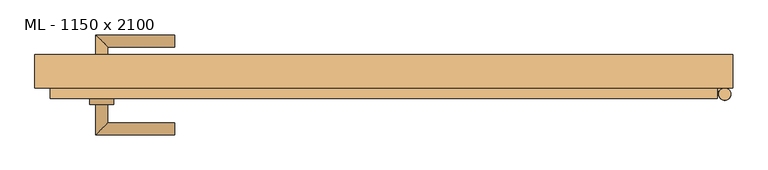
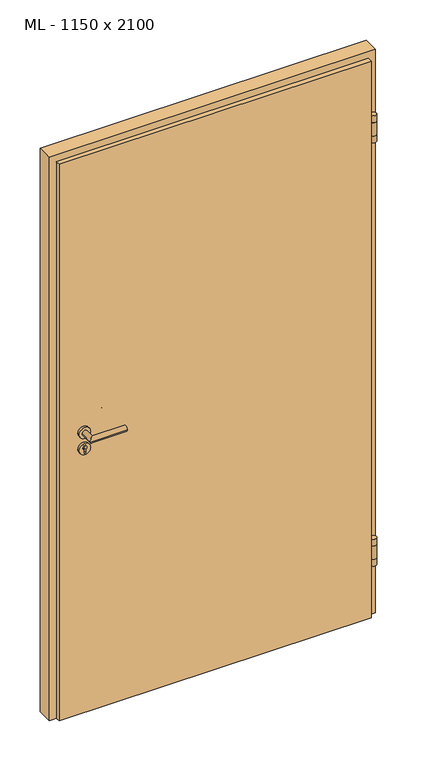
"""IFC4 building model written with IfcOpenShell, lengths in millimetres: door geometry, TU DF 1 - Pfostenstock Falztüre : ML - 1150 x 2100."""

import ifcopenshell
import ifcopenshell.guid

model = None  # the IFC model being written
_history = None  # IfcOwnerHistory: only IFC2X3 demands one
_inside = {}  # id of a spatial element -> (the spatial element, [elements in it])
_under = {}  # id of a project, library or spatial element -> (it, [spatial elements below it])
_declared = {}  # id of a project -> (the project, [libraries it declares])
_typed = {}  # id of a type object -> (the type object, [elements of that type])
_made_of = {}  # id of a material, layer set ... -> (it, [elements and type objects made of it])


def new_model(schema):
    """Start an empty IFC model of exactly this schema.

    Asked for "IFC4X3", IfcOpenShell would pick the latest addendum, in which some entities
    have other attributes; the version numbers below select the first issue.
    IFC2X3 requires an IfcOwnerHistory on every rooted entity: one is made here for all.
    """
    global model, _history
    if schema == "IFC4X3":
        model = ifcopenshell.file(schema_version=(4, 3, 0, 0))
    else:
        model = ifcopenshell.file(schema=schema)
    _inside.clear()
    _under.clear()
    _declared.clear()
    _typed.clear()
    _made_of.clear()
    _history = None
    if model.schema == "IFC2X3":
        org = make("IfcOrganization", Name="unknown")
        user = make(
            "IfcPersonAndOrganization",
            ThePerson=make("IfcPerson", FamilyName="unknown"),
            TheOrganization=org,
        )
        app = make(
            "IfcApplication",
            ApplicationDeveloper=org,
            Version="unknown",
            ApplicationFullName="unknown",
            ApplicationIdentifier="unknown",
        )
        _history = make(
            "IfcOwnerHistory",
            OwningUser=user,
            OwningApplication=app,
            ChangeAction="ADDED",
            CreationDate=0,
        )
    return model


def make(cls, **values):
    """One entity of the class cls with the attributes given. An attribute that is None is left unset."""
    return model.create_entity(
        cls, **{name: value for name, value in values.items() if value is not None}
    )


def rooted(cls, **values):
    """An entity with a GlobalId (a new one), such as an element, a storey or a relation."""
    return make(cls, GlobalId=ifcopenshell.guid.new(), OwnerHistory=_history, **values)


def si_unit(unit_type, name, prefix=None):
    """IfcSIUnit, for example si_unit("LENGTHUNIT", "METRE", prefix="MILLI")."""
    return make("IfcSIUnit", UnitType=unit_type, Prefix=prefix, Name=name)


def assignment(units):
    """IfcUnitAssignment: the units of a project."""
    return None if units is None else make("IfcUnitAssignment", Units=units)


def point(xyz):
    """IfcCartesianPoint."""
    return None if xyz is None else make("IfcCartesianPoint", Coordinates=xyz)


def direction(xyz):
    """IfcDirection."""
    return None if xyz is None else make("IfcDirection", DirectionRatios=xyz)


def frame(location, z_axis=None, x_axis=None):
    """IfcAxis2Placement3D, a coordinate frame: its origin and axes. An axis left out is left unset."""
    return make(
        "IfcAxis2Placement3D",
        Location=point(location),
        Axis=direction(z_axis),
        RefDirection=direction(x_axis),
    )


def frame_2d(location, x_axis=None):
    """IfcAxis2Placement2D, a coordinate frame in the plane: its origin and x axis."""
    return make(
        "IfcAxis2Placement2D", Location=point(location), RefDirection=direction(x_axis)
    )


def origin():
    """The frame at (0, 0, 0) with its axes left unset."""
    return frame((0.0, 0.0, 0.0))


def place(relative_to, where):
    """IfcLocalPlacement: puts the frame where relative to a parent placement (None: the world)."""
    return make(
        "IfcLocalPlacement", PlacementRelTo=relative_to, RelativePlacement=where
    )


def context(
    kind, dimensions, precision=None, world=None, true_north=None, identifier=None
):
    """IfcGeometricRepresentationContext, for example the 3D "Model" context."""
    return make(
        "IfcGeometricRepresentationContext",
        ContextIdentifier=identifier,
        ContextType=kind,
        CoordinateSpaceDimension=dimensions,
        Precision=precision,
        WorldCoordinateSystem=world,
        TrueNorth=true_north,
    )


def project(units=None, contexts=None):
    """IfcProject with its units and contexts."""
    return rooted(
        "IfcProject",
        Name="project",
        RepresentationContexts=contexts,
        UnitsInContext=assignment(units),
    )


def spatial(cls, under=None, at=None, **own):
    """A site, building, storey or space (cls), placed at a placement, below another one or the project."""
    s = rooted(cls, ObjectPlacement=at, **own)
    if under is not None:
        _under.setdefault(under.id(), (under, []))[1].append(s)
    return s


def polyline(points):
    """IfcPolyline through the points."""
    return make("IfcPolyline", Points=[point(p) for p in points])


def circle_curve(where, radius):
    """IfcCircle in the frame where."""
    return make("IfcCircle", Position=where, Radius=radius)


def ellipse_curve(where, semi_axis1, semi_axis2):
    """IfcEllipse in the frame where."""
    return make(
        "IfcEllipse", Position=where, SemiAxis1=semi_axis1, SemiAxis2=semi_axis2
    )


def trimmed(basis, trim1, trim2, sense, master):
    """IfcTrimmedCurve: the piece of a basis curve between two trims."""
    return make(
        "IfcTrimmedCurve",
        BasisCurve=basis,
        Trim1=trim1,
        Trim2=trim2,
        SenseAgreement=sense,
        MasterRepresentation=master,
    )


def segment(curve, same_sense, transition):
    """IfcCompositeCurveSegment."""
    return make(
        "IfcCompositeCurveSegment",
        Transition=transition,
        SameSense=same_sense,
        ParentCurve=curve,
    )


def composite_curve(segments, self_intersect=None):
    """IfcCompositeCurve: segments joined end to end."""
    return make("IfcCompositeCurve", Segments=segments, SelfIntersect=self_intersect)


def outline(outer, holes=None, kind="AREA"):
    """IfcArbitraryClosedProfileDef: a profile drawn as a closed curve; with holes, ...WithVoids."""
    if holes is None:
        return make("IfcArbitraryClosedProfileDef", ProfileType=kind, OuterCurve=outer)
    return make(
        "IfcArbitraryProfileDefWithVoids",
        ProfileType=kind,
        OuterCurve=outer,
        InnerCurves=holes,
    )


def extrude(swept, where, along, depth):
    """IfcExtrudedAreaSolid: the profile swept, set in the frame where, extruded along a direction by depth."""
    return make(
        "IfcExtrudedAreaSolid",
        SweptArea=swept,
        Position=where,
        ExtrudedDirection=direction(along),
        Depth=depth,
    )


def faces_of(points, faces, orient=None, outer=None):
    """IfcFace entities. A face is a list of loops; a loop is a list of indices into points, from 0.

    orient and outer hold one flag for each loop. By default every Orientation is true, the
    first loop of a face is its IfcFaceOuterBound and the others are IfcFaceBound.
    """
    made = []
    for i, loops in enumerate(faces):
        bounds = []
        for j, loop in enumerate(loops):
            is_outer = j == 0 if outer is None else outer[i][j]
            bounds.append(
                make(
                    "IfcFaceOuterBound" if is_outer else "IfcFaceBound",
                    Bound=make("IfcPolyLoop", Polygon=[points[k] for k in loop]),
                    Orientation=True if orient is None else orient[i][j],
                )
            )
        made.append(make("IfcFace", Bounds=bounds))
    return made


def faceted_brep(points, faces, orient=None, outer=None, voids=None):
    """IfcFacetedBrep: a solid bounded by flat faces; with voids (closed shells), ...WithVoids."""
    shared = [point(p) for p in points]
    hull = make("IfcClosedShell", CfsFaces=faces_of(shared, faces, orient, outer))
    if voids is None:
        return make("IfcFacetedBrep", Outer=hull)
    return make(
        "IfcFacetedBrepWithVoids",
        Outer=hull,
        Voids=[
            make(cls, CfsFaces=faces_of(shared, fs, o, b)) for cls, fs, o, b in voids
        ],
    )


def shape(context_of_items, identifier, shape_type, items):
    """IfcShapeRepresentation: the items that make up one representation, for example the "Body"."""
    return make(
        "IfcShapeRepresentation",
        ContextOfItems=context_of_items,
        RepresentationIdentifier=identifier,
        RepresentationType=shape_type,
        Items=items,
    )


def source(mapping_origin, context_of_items, identifier, shape_type, items):
    """IfcRepresentationMap: a shape defined once, which mapped items show again and again."""
    return make(
        "IfcRepresentationMap",
        MappingOrigin=mapping_origin,
        MappedRepresentation=shape(context_of_items, identifier, shape_type, items),
    )


def transform(
    local_origin,
    x_axis=None,
    y_axis=None,
    z_axis=None,
    scale=None,
    scale2=None,
    scale3=None,
    uniform=True,
):
    """IfcCartesianTransformationOperator3D, or its non-uniform kind. x_axis, y_axis, z_axis: its Axis1, 2, 3."""
    if uniform:
        return make(
            "IfcCartesianTransformationOperator3D",
            Axis1=direction(x_axis),
            Axis2=direction(y_axis),
            LocalOrigin=point(local_origin),
            Scale=scale,
            Axis3=direction(z_axis),
        )
    return make(
        "IfcCartesianTransformationOperator3DnonUniform",
        Axis1=direction(x_axis),
        Axis2=direction(y_axis),
        LocalOrigin=point(local_origin),
        Scale=scale,
        Axis3=direction(z_axis),
        Scale2=scale2,
        Scale3=scale3,
    )


def mapped(mapping_source, mapping_target):
    """IfcMappedItem: shows the shape of a source again, moved by a transform."""
    return make(
        "IfcMappedItem", MappingSource=mapping_source, MappingTarget=mapping_target
    )


def made_of(thing, what):
    """Note that an element or type object is made of a material, layer set ...; save() writes the relation."""
    if what is not None:
        _made_of.setdefault(what.id(), (what, []))[1].append(thing)
    return thing


def element(
    cls,
    number,
    at=None,
    inside=None,
    cuts=None,
    type_object=None,
    material=None,
    context=None,
    identifier="Body",
    shape_type=None,
    held_by="IfcProductDefinitionShape",
    body=None,
    shapes=None,
    **own,
):
    """One element of the class cls, such as IfcWall. Its Tag is "e" and its number.

    at: its placement. inside: the storey or other place that contains it. cuts: it is an
    opening in that element (IfcRelVoidsElement). A single representation is given by context,
    identifier, shape_type and body (its items); several are given by shapes. held_by: the class
    of the entity that holds the representations. save() writes the other relations.
    """
    e = rooted(cls, Tag="e%d" % number, ObjectPlacement=at, **own)
    if body is not None:
        shapes = [shape(context, identifier, shape_type, body)]
    if shapes is not None:
        e.Representation = make(held_by, Representations=shapes)
    if inside is not None:
        _inside.setdefault(inside.id(), (inside, []))[1].append(e)
    if cuts is not None:
        rooted(
            "IfcRelVoidsElement", RelatingBuildingElement=cuts, RelatedOpeningElement=e
        )
    if type_object is not None:
        _typed.setdefault(type_object.id(), (type_object, []))[1].append(e)
    return made_of(e, material)


def aggregate(whole, parts):
    """IfcRelAggregates: a whole, such as a stair, and the parts it consists of."""
    return rooted("IfcRelAggregates", RelatingObject=whole, RelatedObjects=parts)


def save(model, path):
    """Write the relations noted so far, then the file.

    IfcRelAggregates (storeys below a building ...), IfcRelContainedInSpatialStructure (elements
    in a storey), IfcRelDefinesByType, IfcRelAssociatesMaterial and IfcRelDeclares: one each for
    every whole, place, type object, material and project.
    """
    for whole, parts in _under.values():
        aggregate(whole, parts)
    for where, things in _inside.values():
        rooted(
            "IfcRelContainedInSpatialStructure",
            RelatedElements=things,
            RelatingStructure=where,
        )
    for kind, things in _typed.values():
        rooted("IfcRelDefinesByType", RelatedObjects=things, RelatingType=kind)
    for what, things in _made_of.values():
        rooted("IfcRelAssociatesMaterial", RelatedObjects=things, RelatingMaterial=what)
    for by, libraries in _declared.values():
        rooted("IfcRelDeclares", RelatingContext=by, RelatedDefinitions=libraries)
    model.write(path)


def plane_surface(at):
    """IfcPlane: the flat surface through the origin of the frame at, square to its z axis."""
    return make("IfcPlane", Position=at)


def cylinder_surface(at, radius):
    """IfcCylindricalSurface: all points at the distance radius from the z axis of the frame at."""
    return make("IfcCylindricalSurface", Position=at, Radius=radius)


def advanced_brep(points, edges, surfaces, faces):
    """IfcAdvancedBrep: a solid bounded by faces that lie on surfaces and meet in shared edges.

    An edge is (start, end): straight between two places in points (the first is 0);
    or (start, end, curve); or (start, end, curve, False) where it runs against its curve.
    A face is (place in surfaces, loops), or (place, loops, False) where it looks against
    its surface's normal. A loop lists edges by number (the first is 1), with a minus sign
    where the edge is run from its end to its start. The first loop is the outer one.
    """
    corners = [point(p) for p in points]
    vertices = [make("IfcVertexPoint", VertexGeometry=c) for c in corners]
    made = []
    for start, end, *more in edges:
        made.append(
            make(
                "IfcEdgeCurve",
                EdgeStart=vertices[start],
                EdgeEnd=vertices[end],
                EdgeGeometry=more[0] if more else make("IfcPolyline", Points=[corners[start], corners[end]]),
                SameSense=more[1] if len(more) > 1 else True,
            )
        )
    hull = []
    for where, loops, *sense in faces:
        bounds = []
        for j, loop in enumerate(loops):
            ring = [make("IfcOrientedEdge", EdgeElement=made[abs(k) - 1], Orientation=k > 0) for k in loop]
            bounds.append(
                make(
                    "IfcFaceOuterBound" if j == 0 else "IfcFaceBound",
                    Bound=make("IfcEdgeLoop", EdgeList=ring),
                    Orientation=True,
                )
            )
        hull.append(make("IfcAdvancedFace", Bounds=bounds, FaceSurface=surfaces[where], SameSense=sense[0] if sense else True))
    return make("IfcAdvancedBrep", Outer=make("IfcClosedShell", CfsFaces=hull))


def ml_1150_x_2100_f64283a4(model_context):
    return source(origin(), model_context, "Body", "SolidModel", [
        faceted_brep([(550.0, -44.5, 0.0), (-550.0, -44.5, 0.0), (-550.0, -27.5, 0.0), (-535.0, -27.5, 0.0), (-535.0, 0.5, 0.0), (535.0, 0.5, 0.0), (535.0, -27.5, 0.0), (550.0, -27.5, 0.0), (550.0, -44.5, 2075.0), (-550.0, -44.5, 2075.0), (-550.0, -27.5, 2075.0), (-535.0, -27.5, 2060.0), (550.0, -27.5, 2075.0), (535.0, -27.5, 2060.0), (-535.0, 0.5, 2060.0), (535.0, 0.5, 2060.0)], [[[0, 1, 2, 3, 4, 5, 6, 7]], [[8, 9, 1, 0]], [[1, 9, 10, 2]], [[11, 3, 2, 10, 12, 7, 6, 13]], [[3, 11, 14, 4]], [[5, 4, 14, 15]], [[13, 6, 5, 15]], [[8, 0, 7, 12]], [[9, 8, 12, 10]], [[11, 13, 15, 14]]]),
        extrude(outline(composite_curve([segment(trimmed(circle_curve(frame_2d((562.0, -37.5)), 10.0), [point((552.0, -37.5))], [point((572.0, -37.5))], False, "CARTESIAN"), True, "CONTINUOUS"), segment(trimmed(circle_curve(frame_2d((562.0, -37.5)), 10.0), [point((572.0, -37.5))], [point((552.0, -37.5))], False, "CARTESIAN"), True, "CONTINUOUS")], self_intersect=False)), frame((0.0, 0.0, 1844.0), z_axis=(0.0, 0.0, 1.0), x_axis=(1.0, 0.0, 0.0)), (0.0, 0.0, 1.0), 25.0),
        extrude(outline(composite_curve([segment(trimmed(circle_curve(frame_2d((562.0, -37.5)), 10.0), [point((562.0, -27.5))], [point((553.339746, -32.5))], False, "CARTESIAN"), True, "CONTINUOUS"), segment(polyline([(553.339746, -32.5), (550.0, -32.5), (550.0, -27.5), (562.0, -27.5)]), True, "CONTINUOUS")], self_intersect=False)), frame((0.0, 0.0, 1794.0), z_axis=(0.0, 0.0, 1.0), x_axis=(1.0, 0.0, 0.0)), (0.0, 0.0, 1.0), 50.0),
        extrude(outline(composite_curve([segment(trimmed(circle_curve(frame_2d((562.0, -37.5)), 10.0), [point((552.0, -37.5))], [point((572.0, -37.5))], False, "CARTESIAN"), True, "CONTINUOUS"), segment(trimmed(circle_curve(frame_2d((562.0, -37.5)), 10.0), [point((572.0, -37.5))], [point((552.0, -37.5))], False, "CARTESIAN"), True, "CONTINUOUS")], self_intersect=False)), frame((0.0, 0.0, 1769.0), z_axis=(0.0, 0.0, 1.0), x_axis=(1.0, 0.0, 0.0)), (0.0, 0.0, 1.0), 25.0),
        extrude(outline(composite_curve([segment(trimmed(circle_curve(frame_2d((562.0, -37.5)), 10.0), [point((552.0, -37.5))], [point((572.0, -37.5))], False, "CARTESIAN"), True, "CONTINUOUS"), segment(trimmed(circle_curve(frame_2d((562.0, -37.5)), 10.0), [point((572.0, -37.5))], [point((552.0, -37.5))], False, "CARTESIAN"), True, "CONTINUOUS")], self_intersect=False)), frame((0.0, 0.0, 266.0), z_axis=(0.0, 0.0, 1.0), x_axis=(1.0, 0.0, 0.0)), (0.0, 0.0, 1.0), 25.0),
        extrude(outline(composite_curve([segment(trimmed(circle_curve(frame_2d((562.0, -37.5)), 10.0), [point((562.0, -27.5))], [point((553.339746, -32.5))], False, "CARTESIAN"), True, "CONTINUOUS"), segment(polyline([(553.339746, -32.5), (550.0, -32.5), (550.0, -27.5), (562.0, -27.5)]), True, "CONTINUOUS")], self_intersect=False)), frame((0.0, 0.0, 216.0), z_axis=(0.0, 0.0, 1.0), x_axis=(1.0, 0.0, 0.0)), (0.0, 0.0, 1.0), 50.0),
        extrude(outline(composite_curve([segment(trimmed(circle_curve(frame_2d((562.0, -37.5)), 10.0), [point((552.0, -37.5))], [point((572.0, -37.5))], False, "CARTESIAN"), True, "CONTINUOUS"), segment(trimmed(circle_curve(frame_2d((562.0, -37.5)), 10.0), [point((572.0, -37.5))], [point((552.0, -37.5))], False, "CARTESIAN"), True, "CONTINUOUS")], self_intersect=False)), frame((0.0, 0.0, 191.0), z_axis=(0.0, 0.0, 1.0), x_axis=(1.0, 0.0, 0.0)), (0.0, 0.0, 1.0), 25.0),
        advanced_brep(
        [(-455.0, -54.5, 1050.0), (-475.0, -54.5, 1050.0), (-475.0, -104.5, 1050.0), (-455.0, -84.5, 1050.0), (-345.0, -84.5, 1050.0), (-345.0, -104.5, 1050.0)],
        [
            (0, 1, circle_curve(frame((-465.0, -54.5, 1050.0), z_axis=(0.0, 1.0, 0.0), x_axis=(-1.0, 0.0, 0.0)), 10.0)),
            (1, 0, circle_curve(frame((-465.0, -54.5, 1050.0), z_axis=(0.0, 1.0, 0.0), x_axis=(-1.0, 0.0, 0.0)), 10.0)),
            (1, 2),
            (2, 3, ellipse_curve(frame((-465.0, -94.5, 1050.0), z_axis=(-0.7071067811865531, 0.7071067811865419, 0.0), x_axis=(0.707106781186542, 0.707106781186553, 0.0)), 14.1421356, 10.0)),
            (3, 0),
            (3, 2, ellipse_curve(frame((-465.0, -94.5, 1050.0), z_axis=(-0.7071067811865531, 0.7071067811865419, 0.0), x_axis=(0.707106781186542, 0.707106781186553, 0.0)), 14.1421356, 10.0)),
            (4, 5, circle_curve(frame((-345.0, -94.5, 1050.0), z_axis=(1.0, 0.0, 0.0), x_axis=(0.0, -1.0, 0.0)), 10.0)),
            (5, 4, circle_curve(frame((-345.0, -94.5, 1050.0), z_axis=(1.0, 0.0, 0.0), x_axis=(0.0, -1.0, 0.0)), 10.0)),
            (2, 5),
            (4, 3),
        ],
        [
            plane_surface(frame((-465.0, -54.5, 1050.0), z_axis=(0.0, 1.0, 0.0), x_axis=(0.0, 0.0, 1.0))),
            cylinder_surface(frame((-465.0, -54.5, 1050.0), z_axis=(0.0, 1.0, 0.0), x_axis=(-1.0, 0.0, 0.0)), 10.0),
            plane_surface(frame((-345.0, -94.5, 1050.0), z_axis=(1.0, 0.0, 0.0), x_axis=(0.0, 0.0, 1.0))),
            cylinder_surface(frame((-465.0, -94.5, 1050.0), z_axis=(-1.0, 0.0, 0.0), x_axis=(0.0, -1.0, 0.0)), 10.0),
        ],
        [
            (0, [[1, 2]]),
            (1, [[3, 4, 5, -2]]),
            (1, [[-5, 6, -3, -1]]),
            (2, [[7, 8]]),
            (3, [[9, -7, 10, -4]]),
            (3, [[-10, -8, -9, -6]]),
        ],
    ),
        extrude(outline(composite_curve([segment(trimmed(circle_curve(frame_2d((990.0, -465.0)), 20.0), [point((990.0, -485.0))], [point((990.0, -445.0))], False, "CARTESIAN"), True, "CONTINUOUS"), segment(trimmed(circle_curve(frame_2d((990.0, -465.0)), 20.0), [point((990.0, -445.0))], [point((990.0, -485.0))], False, "CARTESIAN"), True, "CONTINUOUS")], self_intersect=False), holes=[composite_curve([segment(polyline([(976.4601385, -467.397268), (988.4749012, -467.397268)]), True, "CONTINUOUS"), segment(trimmed(circle_curve(frame_2d((995.0361633, -465.0)), 6.9854888), [point((988.4749012, -467.397268))], [point((988.4749012, -462.602732))], True, "CARTESIAN"), True, "CONTINUOUS"), segment(polyline([(988.4749012, -462.602732), (976.4601385, -462.602732)]), True, "CONTINUOUS"), segment(trimmed(circle_curve(frame_2d((976.4601385, -465.0)), 2.397268), [point((976.4601385, -462.602732))], [point((976.4601385, -467.397268))], True, "CARTESIAN"), True, "CONTINUOUS")], self_intersect=False)]), frame((0.0, -54.5, 0.0), z_axis=(0.0, 1.0, 0.0), x_axis=(0.0, 0.0, 1.0)), (0.0, 0.0, 1.0), 10.0),
        advanced_brep(
        [(-455.0, -54.5, 1050.0), (-475.0, -54.5, 1050.0), (-475.0, -104.5, 1050.0), (-455.0, -84.5, 1050.0), (-345.0, -84.5, 1050.0), (-345.0, -104.5, 1050.0)],
        [
            (0, 1, circle_curve(frame((-465.0, -54.5, 1050.0), z_axis=(0.0, 1.0, 0.0), x_axis=(-1.0, 0.0, 0.0)), 10.0)),
            (1, 0, circle_curve(frame((-465.0, -54.5, 1050.0), z_axis=(0.0, 1.0, 0.0), x_axis=(-1.0, 0.0, 0.0)), 10.0)),
            (1, 2),
            (2, 3, ellipse_curve(frame((-465.0, -94.5, 1050.0), z_axis=(-0.7071067811865537, 0.7071067811865414, 0.0), x_axis=(0.7071067811865414, 0.7071067811865536, 0.0)), 14.1421356, 10.0)),
            (3, 0),
            (3, 2, ellipse_curve(frame((-465.0, -94.5, 1050.0), z_axis=(-0.7071067811865537, 0.7071067811865414, 0.0), x_axis=(0.7071067811865414, 0.7071067811865536, 0.0)), 14.1421356, 10.0)),
            (4, 5, circle_curve(frame((-345.0, -94.5, 1050.0), z_axis=(1.0, 0.0, 0.0), x_axis=(0.0, -1.0, 0.0)), 10.0)),
            (5, 4, circle_curve(frame((-345.0, -94.5, 1050.0), z_axis=(1.0, 0.0, 0.0), x_axis=(0.0, -1.0, 0.0)), 10.0)),
            (2, 5),
            (4, 3),
        ],
        [
            plane_surface(frame((-465.0, -54.5, 1050.0), z_axis=(0.0, 1.0, 0.0), x_axis=(0.0, 0.0, 1.0))),
            cylinder_surface(frame((-465.0, -54.5, 1050.0), z_axis=(0.0, 1.0, 0.0), x_axis=(-1.0, 0.0, 0.0)), 10.0),
            plane_surface(frame((-345.0, -94.5, 1050.0), z_axis=(1.0, 0.0, 0.0), x_axis=(0.0, 0.0, 1.0))),
            cylinder_surface(frame((-465.0, -94.5, 1050.0), z_axis=(-1.0, 0.0, 0.0), x_axis=(0.0, -1.0, 0.0)), 10.0),
        ],
        [
            (0, [[1, 2]]),
            (1, [[3, 4, 5, -2]]),
            (1, [[-5, 6, -3, -1]]),
            (2, [[7, 8]]),
            (3, [[9, -7, 10, -4]]),
            (3, [[-10, -8, -9, -6]]),
        ],
    ),
        extrude(outline(composite_curve([segment(trimmed(circle_curve(frame_2d((1050.0, -465.0)), 20.0), [point((1050.0, -485.0))], [point((1050.0, -445.0))], False, "CARTESIAN"), True, "CONTINUOUS"), segment(trimmed(circle_curve(frame_2d((1050.0, -465.0)), 20.0), [point((1050.0, -445.0))], [point((1050.0, -485.0))], False, "CARTESIAN"), True, "CONTINUOUS")], self_intersect=False)), frame((0.0, -54.5, 0.0), z_axis=(0.0, 1.0, 0.0), x_axis=(0.0, 0.0, 1.0)), (0.0, 0.0, 1.0), 10.0),
        advanced_brep(
        [(-455.0, 10.5, 1050.0), (-475.0, 10.5, 1050.0), (-455.0, 40.5, 1050.0), (-475.0, 60.5, 1050.0), (-345.0, 40.5, 1050.0), (-345.0, 60.5, 1050.0)],
        [
            (0, 1, circle_curve(frame((-465.0, 10.5, 1050.0), z_axis=(0.0, -1.0, 0.0), x_axis=(-1.0, 0.0, 0.0)), 10.0)),
            (1, 0, circle_curve(frame((-465.0, 10.5, 1050.0), z_axis=(0.0, -1.0, 0.0), x_axis=(-1.0, 0.0, 0.0)), 10.0)),
            (0, 2),
            (2, 3, ellipse_curve(frame((-465.0, 50.5, 1050.0), z_axis=(-0.7071067811865486, -0.7071067811865464, 0.0), x_axis=(0.7071067811865464, -0.7071067811865488, 0.0)), 14.1421356, 10.0)),
            (3, 1),
            (3, 2, ellipse_curve(frame((-465.0, 50.5, 1050.0), z_axis=(-0.7071067811865486, -0.7071067811865464, 0.0), x_axis=(0.7071067811865464, -0.7071067811865488, 0.0)), 14.1421356, 10.0)),
            (4, 5, circle_curve(frame((-345.0, 50.5, 1050.0), z_axis=(1.0, 0.0, 0.0), x_axis=(0.0, 1.0, 0.0)), 10.0)),
            (5, 4, circle_curve(frame((-345.0, 50.5, 1050.0), z_axis=(1.0, 0.0, 0.0), x_axis=(0.0, 1.0, 0.0)), 10.0)),
            (2, 4),
            (5, 3),
        ],
        [
            plane_surface(frame((-465.0, 10.5, 1050.0), z_axis=(0.0, -1.0, 0.0), x_axis=(0.0, 0.0, 1.0))),
            cylinder_surface(frame((-465.0, 10.5, 1050.0), z_axis=(0.0, -1.0, 0.0), x_axis=(-1.0, 0.0, 0.0)), 10.0),
            plane_surface(frame((-345.0, 50.5, 1050.0), z_axis=(1.0, 0.0, 0.0), x_axis=(0.0, 0.0, 1.0))),
            cylinder_surface(frame((-465.0, 50.5, 1050.0), z_axis=(-1.0, 0.0, 0.0), x_axis=(0.0, 1.0, 0.0)), 10.0),
        ],
        [
            (0, [[1, 2]]),
            (1, [[-1, 3, 4, 5]]),
            (1, [[-2, -5, 6, -3]]),
            (2, [[7, 8]]),
            (3, [[-4, 9, -8, 10]]),
            (3, [[-6, -10, -7, -9]]),
        ],
    ),
        extrude(outline(composite_curve([segment(trimmed(circle_curve(frame_2d((990.0, -465.0)), 20.0), [point((990.0, -485.0))], [point((990.0, -445.0))], False, "CARTESIAN"), True, "CONTINUOUS"), segment(trimmed(circle_curve(frame_2d((990.0, -465.0)), 20.0), [point((990.0, -445.0))], [point((990.0, -485.0))], False, "CARTESIAN"), True, "CONTINUOUS")], self_intersect=False), holes=[composite_curve([segment(polyline([(976.4601385, -467.397268), (988.4749012, -467.397268)]), True, "CONTINUOUS"), segment(trimmed(circle_curve(frame_2d((995.0361633, -465.0)), 6.9854888), [point((988.4749012, -467.397268))], [point((988.4749012, -462.602732))], True, "CARTESIAN"), True, "CONTINUOUS"), segment(polyline([(988.4749012, -462.602732), (976.4601385, -462.602732)]), True, "CONTINUOUS"), segment(trimmed(circle_curve(frame_2d((976.4601385, -465.0)), 2.397268), [point((976.4601385, -462.602732))], [point((976.4601385, -467.397268))], True, "CARTESIAN"), True, "CONTINUOUS")], self_intersect=False)]), frame((0.0, 0.5, 0.0), z_axis=(0.0, 1.0, 0.0), x_axis=(0.0, 0.0, 1.0)), (0.0, 0.0, 1.0), 10.0),
        advanced_brep(
        [(-455.0, 10.5, 1050.0), (-475.0, 10.5, 1050.0), (-455.0, 40.5, 1050.0), (-475.0, 60.5, 1050.0), (-345.0, 40.5, 1050.0), (-345.0, 60.5, 1050.0)],
        [
            (0, 1, circle_curve(frame((-465.0, 10.5, 1050.0), z_axis=(0.0, -1.0, 0.0), x_axis=(-1.0, 0.0, 0.0)), 10.0)),
            (1, 0, circle_curve(frame((-465.0, 10.5, 1050.0), z_axis=(0.0, -1.0, 0.0), x_axis=(-1.0, 0.0, 0.0)), 10.0)),
            (0, 2),
            (2, 3, ellipse_curve(frame((-465.0, 50.5, 1050.0), z_axis=(-0.7071067811865491, -0.7071067811865459, 0.0), x_axis=(0.7071067811865458, -0.7071067811865492, 0.0)), 14.1421356, 10.0)),
            (3, 1),
            (3, 2, ellipse_curve(frame((-465.0, 50.5, 1050.0), z_axis=(-0.7071067811865491, -0.7071067811865459, 0.0), x_axis=(0.7071067811865458, -0.7071067811865492, 0.0)), 14.1421356, 10.0)),
            (4, 5, circle_curve(frame((-345.0, 50.5, 1050.0), z_axis=(1.0, 0.0, 0.0), x_axis=(0.0, 1.0, 0.0)), 10.0)),
            (5, 4, circle_curve(frame((-345.0, 50.5, 1050.0), z_axis=(1.0, 0.0, 0.0), x_axis=(0.0, 1.0, 0.0)), 10.0)),
            (2, 4),
            (5, 3),
        ],
        [
            plane_surface(frame((-465.0, 10.5, 1050.0), z_axis=(0.0, -1.0, 0.0), x_axis=(0.0, 0.0, 1.0))),
            cylinder_surface(frame((-465.0, 10.5, 1050.0), z_axis=(0.0, -1.0, 0.0), x_axis=(-1.0, 0.0, 0.0)), 10.0),
            plane_surface(frame((-345.0, 50.5, 1050.0), z_axis=(1.0, 0.0, 0.0), x_axis=(0.0, 0.0, 1.0))),
            cylinder_surface(frame((-465.0, 50.5, 1050.0), z_axis=(-1.0, 0.0, 0.0), x_axis=(0.0, 1.0, 0.0)), 10.0),
        ],
        [
            (0, [[1, 2]]),
            (1, [[-1, 3, 4, 5]]),
            (1, [[-2, -5, 6, -3]]),
            (2, [[7, 8]]),
            (3, [[-4, 9, -8, 10]]),
            (3, [[-6, -10, -7, -9]]),
        ],
    ),
        extrude(outline(composite_curve([segment(trimmed(circle_curve(frame_2d((1050.0, -465.0)), 20.0), [point((1050.0, -485.0))], [point((1050.0, -445.0))], False, "CARTESIAN"), True, "CONTINUOUS"), segment(trimmed(circle_curve(frame_2d((1050.0, -465.0)), 20.0), [point((1050.0, -445.0))], [point((1050.0, -485.0))], False, "CARTESIAN"), True, "CONTINUOUS")], self_intersect=False)), frame((0.0, 0.5, 0.0), z_axis=(0.0, 1.0, 0.0), x_axis=(0.0, 0.0, 1.0)), (0.0, 0.0, 1.0), 10.0),
        faceted_brep([(-535.0, -27.5, 0.0), (-575.0, -27.5, 0.0), (-575.0, 27.5, 0.0), (-520.0, 27.5, 0.0), (-520.0, 0.5, 0.0), (-535.0, 0.5, 0.0), (-535.0, 0.5, 2060.0), (-535.0, -27.5, 2060.0), (-520.0, 0.5, 2045.0), (520.0, 0.5, 2045.0), (520.0, 0.5, 0.0), (535.0, 0.5, 0.0), (535.0, 0.5, 2060.0), (-520.0, 27.5, 2045.0), (-575.0, 27.5, 2100.0), (575.0, 27.5, 2100.0), (575.0, 27.5, 0.0), (520.0, 27.5, 0.0), (520.0, 27.5, 2045.0), (-575.0, -27.5, 2100.0), (535.0, -27.5, 2060.0), (535.0, -27.5, 0.0), (575.0, -27.5, 0.0), (575.0, -27.5, 2100.0)], [[[0, 1, 2, 3, 4, 5]], [[5, 6, 7, 0]], [[4, 8, 9, 10, 11, 12, 6, 5]], [[3, 13, 8, 4]], [[2, 14, 15, 16, 17, 18, 13, 3]], [[1, 19, 14, 2]], [[0, 7, 20, 21, 22, 23, 19, 1]], [[23, 22, 16, 15]], [[21, 11, 10, 17, 16, 22]], [[12, 11, 21, 20]], [[18, 17, 10, 9]], [[19, 23, 15, 14]], [[13, 18, 9, 8]], [[6, 12, 20, 7]]]),
    ])


if __name__ == "__main__":
    model = new_model("IFC4")
    model_context = context("Model", 3, world=origin())
    ifc_project = project(units=[si_unit("LENGTHUNIT", "METRE", prefix="MILLI")], contexts=[model_context])
    site = spatial("IfcSite", under=ifc_project)
    building = spatial("IfcBuilding", under=site)
    placement = place(None, origin())
    ml_1150_x_2100_shape = ml_1150_x_2100_f64283a4(model_context)
    element("IfcDoor", 1, ObjectType="TU DF 1 - Pfostenstock Falztüre : ML - 1150 x 2100", at=placement, inside=building, context=model_context, shape_type="MappedRepresentation", body=[
        mapped(ml_1150_x_2100_shape, transform((0.0, 0.0, 0.0), x_axis=(1.0, 0.0, 0.0), y_axis=(0.0, 1.0, 0.0), z_axis=(0.0, 0.0, 1.0))),
    ])
    save(model, "model.ifc")

# Revit data of these elements
# Type "TU DF 1 - Pfostenstock Falztüre : ML - 1150 x 2100"
#   Type IfcGUID = "32vBIxahr8bQdQw1D1hUYB"
#   Type Mark = "234"
#   Operation = "SINGLE_SWING_RIGHT"
#   URL = "http://www.autodesk.de/BIM"
#   Type Comments = "Pfostenstock Falztüre"
#   Form Tür = "rechteckig"
#   Description = "1-teilig"
#   Ausführung Zarge = "Blockzarge"
#   Anzahl Seitenteile = "0"
#   Anzahl Oberlichter = "0"
#   Anzahl Flügel = "einflügelig"
#   Anschlag- / Bewegungsart Tür = "Drehflügeltür"
#   Analytic Construction = "<Keine Auswahl>"
#   Winkel Öffnungsbogen [instance default] = 90.00°
#   Wandstärke Gesamt [instance default] = 0.300 m
#   Wandstärke [instance default] = 0.300 m
#   Wandaufbau Gegenbandseite [instance default] = 0.000 m
#   Wandaufbau Bandseite [instance default] = 0.000 m
#   Rough Height [instance default] = 2.280 m
#   Rough Width = 1.150 m
#   Randabstand Öffnungssymbol = 0.000 m
#   Rahmentiefe = 0.055 m
#   Rahmendicke = 0.055 m
#   Höhe ab FBOK = 2.100 m
#   Fußbodenaufbau [instance default] = 0.180 m
#   Height [instance default] = 2.100 m
#   Falztiefe = 0.028 m
#   Falzaufschlag = 0.017 m
#   Einbautiefe [instance default] = 0.080 m
#   Durchgangshöhe = 2.045 m
#   Durchgangsbreite = 1.040 m
#   Drückerhöhe = 1.050 m
#   Thickness = 0.045 m
#   Width = 1.150 m
#   B_Einbautiefe [instance default] = 0.1225 m
#   Angabe Maueröffnungsmaß Höhe = 2.100 m
#   Angabe Maueröffnungsmaß Breite = 1.150 m
#   Angabe Lichter Durchgang Höhe = 2.000 m
#   Angabe Lichter Durchgang Breite = 0.800 m
#   Zylinderrosette [instance default] = yes
#   Tür mit Anschlag [instance default] = no
#   Pfostenstock Wandmittig eingebaut [instance default] = yes
#   Kollisionskörper einschalten [instance default] = no
#   Knauf Innenseite [instance default] = no
#   Knauf Außenseite [instance default] = no
#   Höhe ab FBOK berechnen = yes
#   Größenberechnung über Maueröffnungsmaß = yes
#   Größenberechnung über Lichten Durchgang = no
#   Grundrissdarstellung Türsturz [instance default] = no
#   Drücker Bandseite [instance default] = yes
#   Drücker Gegenbandseite [instance default] = yes
#   Türblatt [instance default] = none
#   Sichtbeschläge [instance default] = none
#   Rahmen vertikal [instance default] = none
#   Rahmen horizontal [instance default] = none
#   Kollisionskörper [instance default] = none
#   Function = (empty or 0)
#   Wall Closure = (empty or 0)
#   Fire Rating = ""
# Element 1 (IfcDoor, "TU DF 1 - Pfostenstock Falztüre : ML - 1150 x 2100")
#   Wandstärke Gesamt = 0.120 m
#   Wandstärke = 0.120 m
#   Rough Height = 2.100 m
#   Fußbodenaufbau = 0.000 m
#   B_Einbautiefe = 0.0325 m
#   Türblatt = Holz
#   Rahmen vertikal = Holz
#   Rahmen horizontal = Holz
#   Materials on its faces: "Metall - Edelstahl gebürstet", "Holz"
# Materials
#   "Metall - Edelstahl gebürstet": class "Metall", colour RGB 203 203 203, transparency 0, Description = "Edelstahl gebürstet", Cost = 0
#   "Holz": class "Holz", colour RGB 218 191 173, transparency 0, Description = "Holz - C 20 Cl.1", Cost = 0
